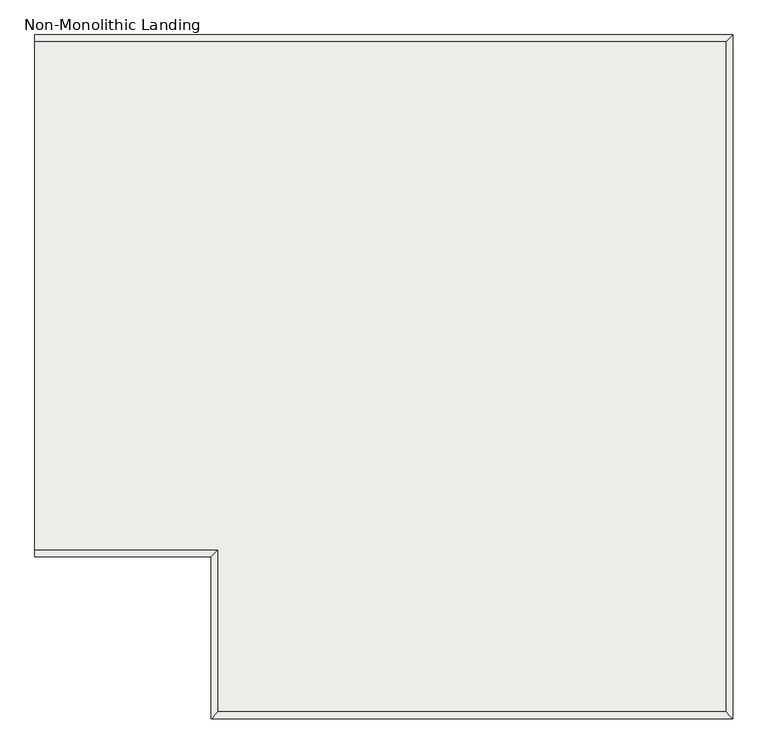
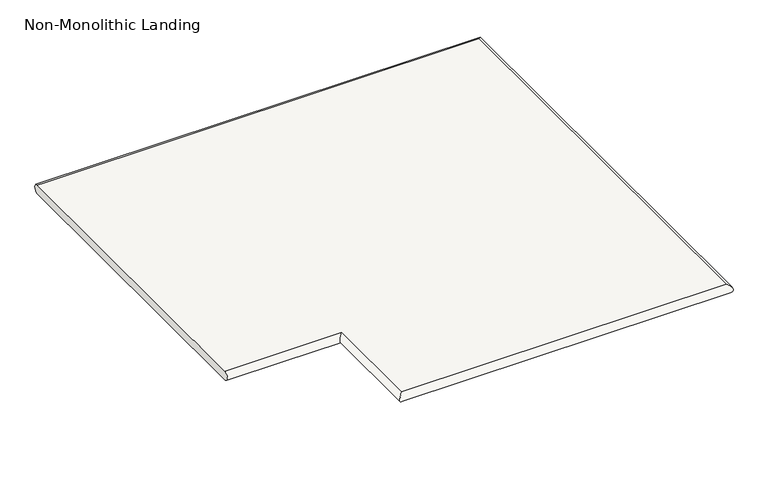
"""IFC4 building model written with IfcOpenShell, lengths in millimetres: slab geometry, Non-Monolithic Landing."""

from ifc_helpers import new_model, si_unit, frame, origin, place, context, project, spatial, circle_curve, ellipse_curve, source, transform, mapped, element, save
from ifc_brep_helpers import plane_surface, cylinder_surface, advanced_brep


def non_monolithic_landing_288ef07f(model_context):
    return source(origin(), model_context, "Body", "AdvancedBrep", [
        advanced_brep(
        [(-6869.5581077, -8654.133999, 1667.9333333), (-6869.5581077, -8654.133999, 1693.3333333), (-7783.9581077, -8654.133999, 1693.3333333), (-7783.9581077, -8654.133999, 1667.9333333), (-8114.1581077, -7447.633999, 1693.3333333), (-8114.1581077, -8362.033999, 1693.3333333), (-8088.7581077, -8362.033999, 1693.3333333), (-7783.9581077, -8362.033999, 1693.3333333), (-6869.5581077, -7447.633999, 1693.3333333), (-8088.7581077, -7447.633999, 1693.3333333), (-8114.1581077, -8362.033999, 1667.9333333), (-8114.1581077, -7447.633999, 1667.9333333), (-8088.7581077, -7447.633999, 1667.9333333), (-6869.5581077, -7447.633999, 1667.9333333), (-7783.9581077, -8362.033999, 1667.9333333), (-8088.7581077, -8362.033999, 1667.9333333)],
        [
            (0, 1, ellipse_curve(frame((-6869.5581077, -8654.133999, 1680.6333333), z_axis=(-0.7071067811865475, -0.7071067811865475, 0.0), x_axis=(0.7071067811865476, -0.7071067811865474, 0.0)), 17.9605122, 12.7)),
            (1, 2),
            (2, 3, ellipse_curve(frame((-7783.9581077, -8654.133999, 1680.6333333), z_axis=(0.7071067811865475, -0.7071067811865475, 0.0), x_axis=(0.7071067811865476, 0.7071067811865474, 0.0)), 17.9605122, 12.7)),
            (3, 0),
            (4, 5),
            (5, 6),
            (6, 7),
            (7, 2),
            (1, 8),
            (8, 9),
            (9, 4),
            (10, 11),
            (11, 12),
            (12, 13),
            (13, 0),
            (3, 14),
            (14, 15),
            (15, 10),
            (4, 11, circle_curve(frame((-8114.1581077, -7447.633999, 1680.6333333), z_axis=(-1.0, 0.0, 0.0), x_axis=(0.0, -1.0, 0.0)), 12.7)),
            (10, 5, circle_curve(frame((-8114.1581077, -8362.033999, 1680.6333333), z_axis=(-1.0, 0.0, 0.0), x_axis=(0.0, 1.0, 0.0)), 12.7)),
            (8, 13, ellipse_curve(frame((-6869.5581077, -7447.633999, 1680.6333333), z_axis=(-0.7071067811865464, 0.7071067811865487, 0.0), x_axis=(-0.7071067811865487, -0.7071067811865464, 0.0)), 17.9605122, 12.7)),
            (7, 14, ellipse_curve(frame((-7783.9581077, -8362.033999, 1680.6333333), z_axis=(0.7071067811865462, -0.7071067811865488, 0.0), x_axis=(-0.7071067811865488, -0.7071067811865462, 0.0)), 17.9605122, 12.7)),
        ],
        [
            cylinder_surface(frame((-6869.5581077, -8654.133999, 1680.6333333), z_axis=(1.0, 0.0, 0.0), x_axis=(0.0, 1.0, 0.0)), 12.7),
            plane_surface(frame((-7783.9581077, -8654.133999, 1693.3333333), z_axis=(0.0, 0.0, 1.0), x_axis=(1.0, 0.0, 0.0))),
            plane_surface(frame((-7783.9581077, -8654.133999, 1667.9333333), z_axis=(0.0, 0.0, -1.0), x_axis=(-1.0, 0.0, 0.0))),
            plane_surface(frame((-8114.1581077, -7447.633999, 1693.3333333), z_axis=(-1.0, 0.0, 0.0), x_axis=(0.0, 0.0, -1.0))),
            cylinder_surface(frame((-8114.1581077, -7447.633999, 1680.6333333), z_axis=(-1.0, 0.0, 0.0), x_axis=(0.0, -1.0, 0.0)), 12.7),
            cylinder_surface(frame((-6869.5581077, -7447.633999, 1680.6333333), z_axis=(0.0, 1.0, 0.0), x_axis=(-1.0, 0.0, 0.0)), 12.7),
            cylinder_surface(frame((-7783.9581077, -8654.133999, 1680.6333333), z_axis=(0.0, -1.0, 0.0), x_axis=(1.0, 0.0, 0.0)), 12.7),
            cylinder_surface(frame((-7783.9581077, -8362.033999, 1680.6333333), z_axis=(1.0, 0.0, 0.0), x_axis=(0.0, 1.0, 0.0)), 12.7),
        ],
        [
            (0, [[1, 2, 3, 4]]),
            (1, [[5, 6, 7, 8, -2, 9, 10, 11]]),
            (2, [[12, 13, 14, 15, -4, 16, 17, 18]]),
            (3, [[-5, 19, -12, 20]]),
            (4, [[-19, -11, -10, 21, -14, -13]]),
            (5, [[-21, -9, -1, -15]]),
            (6, [[-3, -8, 22, -16]]),
            (7, [[-22, -7, -6, -20, -18, -17]]),
        ],
    ),
    ])


if __name__ == "__main__":
    model = new_model("IFC4")
    model_context = context("Model", 3, world=origin())
    ifc_project = project(units=[si_unit("LENGTHUNIT", "METRE", prefix="MILLI")], contexts=[model_context])
    site = spatial("IfcSite", under=ifc_project)
    building = spatial("IfcBuilding", under=site)
    placement = place(None, origin())
    non_monolithic_landing_shape = non_monolithic_landing_288ef07f(model_context)
    element("IfcSlab", 1, ObjectType="Non-Monolithic Landing", at=placement, inside=building, context=model_context, shape_type="MappedRepresentation", body=[
        mapped(non_monolithic_landing_shape, transform((0.0, 0.0, 0.0), x_axis=(1.0, 0.0, 0.0), y_axis=(0.0, 1.0, 0.0), z_axis=(0.0, 0.0, 1.0))),
    ])
    save(model, "model.ifc")

# Revit data of these elements
# Element 1 (IfcSlab, "Non-Monolithic Landing")
#   Materials on its faces: "Wood - Cherry"
# Materials
#   "Wood - Cherry": class "Unassigned", colour RGB 226 177 128, transparency 0
